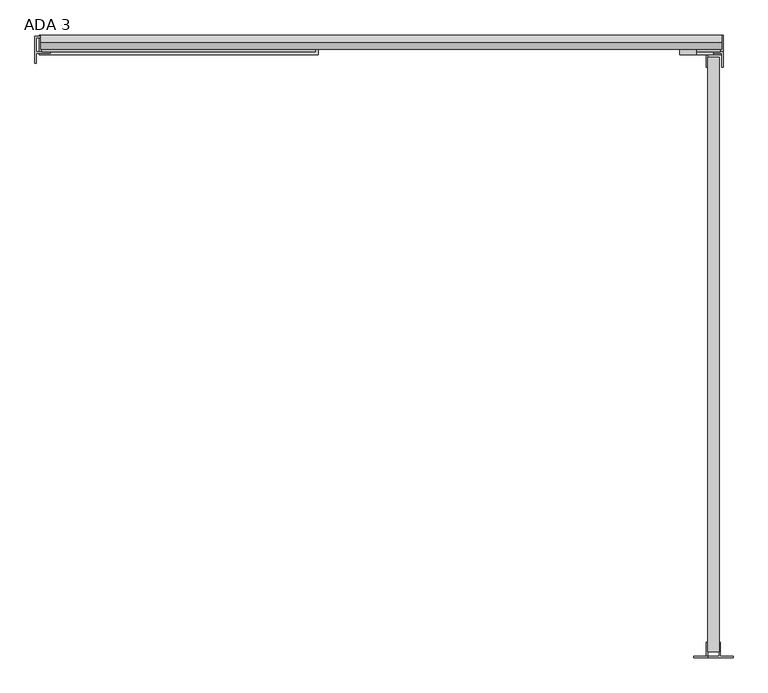
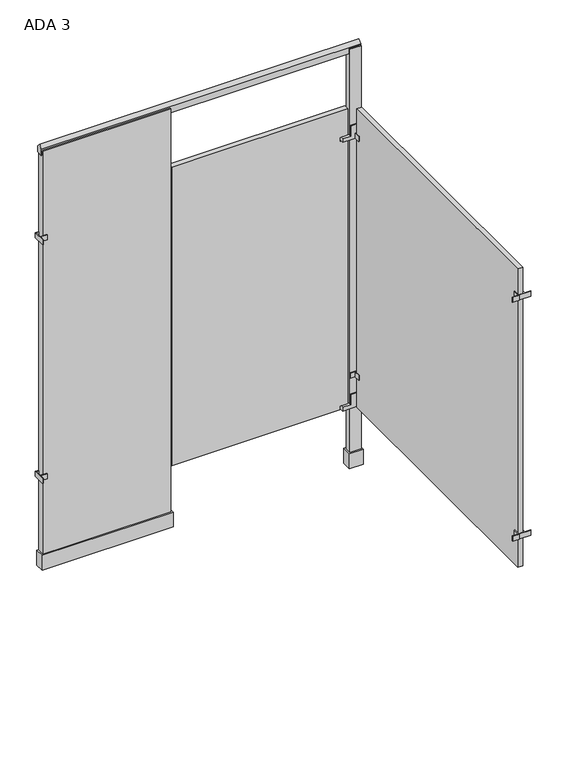
"""IFC4 building model written with IfcOpenShell, lengths in millimetres: proxy geometry, Toilet-Partition_Spec-Rite_Floor-Supported_Headrail : ADA 3."""

from ifc_helpers import new_model, si_unit, frame, origin, origin_with_axes, place, context, project, spatial, polyline, outline, extrude, source, transform, mapped, element, save


def ada_3_4b806e62(model_context):
    return source(origin(), model_context, "Body", "SweptSolid", [
        extrude(outline(polyline([(-94.5439128, 2124.0802205), (-94.5439128, 2092.3302205), (-62.8871683, 2092.3302205), (-62.8871683, 2089.1552205), (-94.5886461, 2089.1552205), (-94.5886461, 2066.9302205), (-97.7189128, 2066.9302205), (-97.7189128, 2127.2552205), (-62.8871683, 2127.2552205), (-62.8871683, 2124.0802205), (-94.5439128, 2124.0802205)])), frame((0.0, 0.0, 1676.4), z_axis=(0.0, 0.0, 1.0), x_axis=(1.0, 0.0, 0.0)), (0.0, 0.0, 1.0), 25.4),
        extrude(outline(polyline([(-94.5439128, 2124.0802205), (-94.5439128, 2092.3302205), (-62.8871683, 2092.3302205), (-62.8871683, 2089.1552205), (-94.5886461, 2089.1552205), (-94.5886461, 2066.9302205), (-97.7189128, 2066.9302205), (-97.7189128, 2127.2552205), (-62.8871683, 2127.2552205), (-62.8871683, 2124.0802205), (-94.5439128, 2124.0802205)])), frame((0.0, 0.0, 457.2), z_axis=(0.0, 0.0, 1.0), x_axis=(1.0, 0.0, 0.0)), (0.0, 0.0, 1.0), 25.4),
        extrude(outline(polyline([(1394.5310872, 720.7302205), (1394.5310872, 723.9052205), (1426.2810872, 723.9052205), (1426.2810872, 720.7302205), (1394.5310872, 720.7302205)])), frame((0.0, 0.0, 1676.4), z_axis=(0.0, 0.0, 1.0), x_axis=(1.0, 0.0, 0.0)), (0.0, 0.0, 1.0), 25.4),
        extrude(outline(polyline([(1426.2810872, 723.9052205), (1451.6810872, 723.9052205), (1451.6810872, 755.561965), (1454.8560872, 755.561965), (1454.8560872, 723.8604872), (1483.4310872, 723.8604872), (1483.4310872, 720.7302205), (1423.1060872, 720.7302205), (1423.1060872, 755.561965), (1426.2810872, 755.561965), (1426.2810872, 723.9052205)])), frame((0.0, 0.0, 1676.4), z_axis=(0.0, 0.0, 1.0), x_axis=(1.0, 0.0, 0.0)), (0.0, 0.0, 1.0), 25.4),
        extrude(outline(polyline([(1394.5310872, 720.7302205), (1394.5310872, 723.9052205), (1426.2810872, 723.9052205), (1426.2810872, 720.7302205), (1394.5310872, 720.7302205)])), frame((0.0, 0.0, 457.2), z_axis=(0.0, 0.0, 1.0), x_axis=(1.0, 0.0, 0.0)), (0.0, 0.0, 1.0), 25.4),
        extrude(outline(polyline([(1426.2810872, 723.9052205), (1451.6810872, 723.9052205), (1451.6810872, 755.561965), (1454.8560872, 755.561965), (1454.8560872, 723.8604872), (1483.4310872, 723.8604872), (1483.4310872, 720.7302205), (1423.1060872, 720.7302205), (1423.1060872, 755.561965), (1426.2810872, 755.561965), (1426.2810872, 723.9052205)])), frame((0.0, 0.0, 457.2), z_axis=(0.0, 0.0, 1.0), x_axis=(1.0, 0.0, 0.0)), (0.0, 0.0, 1.0), 25.4),
        extrude(outline(polyline([(1458.0310872, 2089.1552205), (1426.2810872, 2089.1552205), (1426.2810872, 2057.498476), (1423.1060872, 2057.498476), (1423.1060872, 2089.1999537), (1400.8810872, 2089.1999537), (1400.8810872, 2092.3302205), (1461.2060872, 2092.3302205), (1461.2060872, 2057.498476), (1458.0310872, 2057.498476), (1458.0310872, 2089.1552205)])), frame((0.0, 0.0, 1676.4), z_axis=(0.0, 0.0, 1.0), x_axis=(1.0, 0.0, 0.0)), (0.0, 0.0, 1.0), 25.4),
        extrude(outline(polyline([(1458.0310872, 2089.1552205), (1426.2810872, 2089.1552205), (1426.2810872, 2057.498476), (1423.1060872, 2057.498476), (1423.1060872, 2089.1999537), (1400.8810872, 2089.1999537), (1400.8810872, 2092.3302205), (1461.2060872, 2092.3302205), (1461.2060872, 2057.498476), (1458.0310872, 2057.498476), (1458.0310872, 2089.1552205)])), frame((0.0, 0.0, 457.2), z_axis=(0.0, 0.0, 1.0), x_axis=(1.0, 0.0, 0.0)), (0.0, 0.0, 1.0), 25.4),
        extrude(outline(polyline([(1426.2810872, 2079.6302205), (1451.6810872, 2079.6302205), (1451.6810872, 733.4302205), (1426.2810872, 733.4302205), (1426.2810872, 2079.6302205)])), frame((0.0, 0.0, 304.8), z_axis=(0.0, 0.0, 1.0), x_axis=(1.0, 0.0, 0.0)), (0.0, 0.0, 1.0), 1524.0),
        extrude(outline(polyline([(1454.8560872, 2124.0802205), (1454.8560872, 2092.3302205), (1400.8810872, 2092.3302205), (1400.8810872, 2124.0802205), (1454.8560872, 2124.0802205)])), origin_with_axes(), (0.0, 0.0, 1.0), 2133.6),
        extrude(outline(polyline([(537.2810872, 2124.0802205), (537.2810872, 2092.3302205), (-81.8439128, 2092.3302205), (-81.8439128, 2124.0802205), (537.2810872, 2124.0802205)])), origin_with_axes(), (0.0, 0.0, 1.0), 2133.6),
        extrude(outline(polyline([(499.1810872, 2130.4302205), (562.6810872, 2130.4302205), (562.6810872, 2124.0802205), (499.1810872, 2124.0802205), (499.1810872, 2130.4302205)])), frame((0.0, 0.0, 1015.4167184), z_axis=(0.0, 0.0, 1.0), x_axis=(1.0, 0.0, 0.0)), (0.0, 0.0, 1.0), 51.9665631),
        extrude(outline(polyline([(374.65, 1438.9810872), (374.65, 1400.8810872), (323.85, 1400.8810872), (323.85, 1362.7810872), (304.8, 1362.7810872), (304.8, 1438.9810872), (374.65, 1438.9810872)])), frame((0.0, 2085.9944356, 0.0), z_axis=(0.0, 1.0, 0.0), x_axis=(0.0, 0.0, 1.0)), (0.0, 0.0, 1.0), 44.4357849),
        extrude(outline(polyline([(1746.25, 1438.9810872), (1746.25, 1400.8810872), (1695.45, 1400.8810872), (1695.45, 1362.7810872), (1676.4, 1362.7810872), (1676.4, 1400.8810872), (1676.4, 1438.9810872), (1746.25, 1438.9810872)])), frame((0.0, 2085.9944356, 0.0), z_axis=(0.0, 1.0, 0.0), x_axis=(0.0, 0.0, 1.0)), (0.0, 0.0, 1.0), 44.4357849),
        extrude(outline(polyline([(304.8, 543.6310872), (304.8, 1356.4310872), (323.85, 1356.4310872), (323.85, 1394.5310872), (1674.426485, 1394.5310872), (1674.426485, 1356.4310872), (1695.45, 1356.4310872), (1695.45, 1394.5310872), (1828.8, 1394.5310872), (1828.8, 543.6310872), (304.8, 543.6310872)])), frame((0.0, 2098.6802205, 0.0), z_axis=(0.0, 1.0, 0.0), x_axis=(0.0, 0.0, 1.0)), (0.0, 0.0, 1.0), 25.4),
        extrude(outline(polyline([(2130.4302205, 2139.95), (2130.4302205, 2108.2), (2098.6802205, 2108.2), (2098.6802205, 2139.95), (2114.5552205, 2155.825), (2130.4302205, 2139.95)])), frame((-84.3931269, 0.0, 0.0), z_axis=(1.0, 0.0, 0.0), x_axis=(0.0, 1.0, 0.0)), (0.0, 0.0, 1.0), 1541.9489485),
        extrude(outline(polyline([(1394.5310872, 2130.6646735), (1461.2060872, 2130.6646735), (1461.2060872, 2085.9944356), (1394.5310872, 2085.9944356), (1394.5310872, 2130.6646735)])), origin_with_axes(), (0.0, 0.0, 1.0), 76.2),
        extrude(outline(polyline([(-88.1939128, 2130.304606), (543.6310872, 2130.304606), (543.6310872, 2086.0391689), (-88.1939128, 2086.0391689), (-88.1939128, 2130.304606)])), origin_with_axes(), (0.0, 0.0, 1.0), 76.2),
    ])


if __name__ == "__main__":
    model = new_model("IFC4")
    model_context = context("Model", 3, world=origin())
    ifc_project = project(units=[si_unit("LENGTHUNIT", "METRE", prefix="MILLI")], contexts=[model_context])
    site = spatial("IfcSite", under=ifc_project)
    building = spatial("IfcBuilding", under=site)
    placement = place(None, origin())
    ada_3_shape = ada_3_4b806e62(model_context)
    element("IfcBuildingElementProxy", 1, Name="Toilet-Partition_Spec-Rite_Floor-Supported_Headrail : ADA 3", ObjectType="Toilet-Partition_Spec-Rite_Floor-Supported_Headrail : ADA 3", at=placement, inside=building, context=model_context, shape_type="MappedRepresentation", body=[
        mapped(ada_3_shape, transform((0.0, 0.0, 0.0), x_axis=(1.0, 0.0, 0.0), y_axis=(0.0, 1.0, 0.0), z_axis=(0.0, 0.0, 1.0))),
    ])
    save(model, "model.ifc")

# Revit data of these elements
# Type "Toilet-Partition_Spec-Rite_Floor-Supported_Headrail : ADA 3"
#   URL = "http://www.specritedesigns.com/"
#   UL Fire Rating [instance default] = ""
#   Manufacturer Phone - Toll Free = "877-249-6864"
#   Installation-Fabrication = "http://www.specritedesigns.com/partition_systems.aspx"
#   Green Building-LEED = "http://www.arcat.com/green/clients/leed_data_43944.html"
#   Specification = "http://www.arcat.com/sdspecs/htm/10150you.htm"
#   Send Message = "http://www.arcat.com/users.pl?action=UserEmail&company=Spec-Rite%20Designs%20LLC&coid=43944&rep=146&fax=314-771-4597&mf="
#   Sales Information = "http://www.specritedesigns.com/local_rep.aspx"
#   Revision = "R1_04/2010"
#   Product Properties = "http://www.arcat.com/bim/bim_info.pl?fn=Toilet-Partition_Spec-Rite_"
#   Product Data = "http://www.arcat.com/arcatcos/cos43/arc43944.html"
#   Model = "As Specified in 10 21 13"
#   Manufacturer's Notes = ""
#   Manufacturer Website = "http://www.specritedesigns.com/"
#   Manufacturer Phone = ""
#   Manufacturer Fax = "314-771-4597"
#   Manufacturer Address = "1054 Central Industrial Dr.; St. Louis; MO 63110"
#   Manufacturer = "Spec-Rite Designs LLC"
#   Keynote = "10 21 13"
#   Installation Phase = ""
#   Drawn By = "Robert S. Weygant, CSI, CDT, SCIP"
#   Core Material [instance default] = ""
#   Copyright = "2010, ARCAT, Inc."
#   Description = "As Specified in 10 21 13"
#   Construction Details = "http://www.specritedesigns.com/LinkClick.aspx?fileticket=c2fn%2bPpDPB4%3d&tabid=106"
#   Assembly Code = "C1010400"
#   topoffset = 0' - 0 1/4"
#   hngpnlconstrain [instance default] = 0' - 2 1/8"
#   hngpnl2 [instance default] = 0' - 1 1/8"
#   capoffset = 0' - 0 1/4"
#   Stile Thickness = 0' - 1 1/4"
#   Stall Width = 4' - 11"
#   Stall Depth = 4' - 7 1/4"
#   Pilaster Height = 7' - 0"
#   Panel Thickness = 0' - 1"
#   Panel Height = 5' - 0"
#   Front Panel Width_Strike Side = 2' - 0"
#   Reveal Clearance = 0' - 0 1/2"
#   Front Panel Width_Hinge Side = 0' - 1"
#   Door Width = 2' - 10"
#   Door Thickness = 0' - 1"
#   Distance from Floor to Panel = 1' - 0"
#   strkhdwr [instance default] = no
#   Warranty Duration (Years) = 0
#   Terminates at Wall_Strike Side [instance default] = no
#   Terminates at Wall_Hinge Side [instance default] = no
#   Return Rail - Strike Side [instance default] = yes
#   Return Rail - Hinge Side [instance default] = yes
#   Outswing [instance default] = no
#   Inswing [instance default] = yes
#   End Panel_Strike Side [instance default] = yes
#   Maintenance Schedule (Months) = 0
#   End Panel_Hinge Side [instance default] = yes
#   Expected Lifespan (Years) = 0
#   Brackets_Vertical = 2
#   Headrail Material = Aluminum - Extruded - Satin Anodized Finish
#   Hardware Type [instance default] = element 529356
#   Panel Material [instance default] = Phenolic Core - Color as Specified
#   Hardware Finish [instance default] = Stainless Steel - Type 304 #4 Brushed Finish
#   Type Comments = ""
# Element 1 (IfcBuildingElementProxy, "Toilet-Partition_Spec-Rite_Floor-Supported_Headrail : ADA 3")
#   hngpnl2 = 0' - 0 3/8"
#   Terminates at Wall_Strike Side = yes
#   Return Rail - Strike Side = no
#   Return Rail - Hinge Side = no
#   Outswing = yes
#   Inswing = no
#   End Panel_Strike Side = no
#   Materials on its faces: "Stainless Steel - Type 304 #4 Brushed Finish", "Phenolic Core - Color as Specified", "Aluminum - Extruded - Satin Anodized Finish"
# Materials
#   "Aluminum - Extruded - Satin Anodized Finish": class "Hardware Finishes", colour RGB 244 244 244, transparency 0, Model = "Aluminum - Extruded - Satin Anodized Finish", Description = "Aluminum - Extruded - Satin Anodized Finish", Cost = 0
#   "Phenolic Core - Color as Specified": class "Spec-Rite Partition Finishes", colour RGB 215 199 171, transparency 0, Keynote = "10 21 00", Model = "Phenolic Core - Color as Specified in 10 21 00", Manufacturer = "Spec-Rite Designs LLC", URL = "http://www.specritedesigns.com/", Description = "Phenolic Core - Color as Specified in 10 21 00", Cost = 0
#   "Stainless Steel - Type 304 #4 Brushed Finish": class "Hardware Finishes", colour RGB 189 187 185, transparency 0, Model = "Stainless Steel - Type 304 #4 Brushed Finish", Description = "Stainless Steel - Type 304 #4 Brushed Finish", Cost = 0
